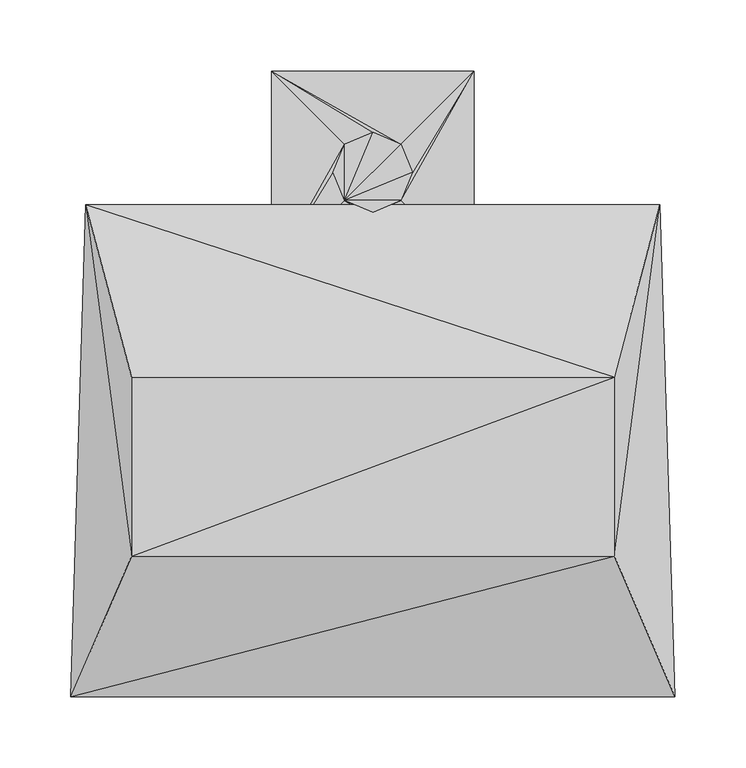
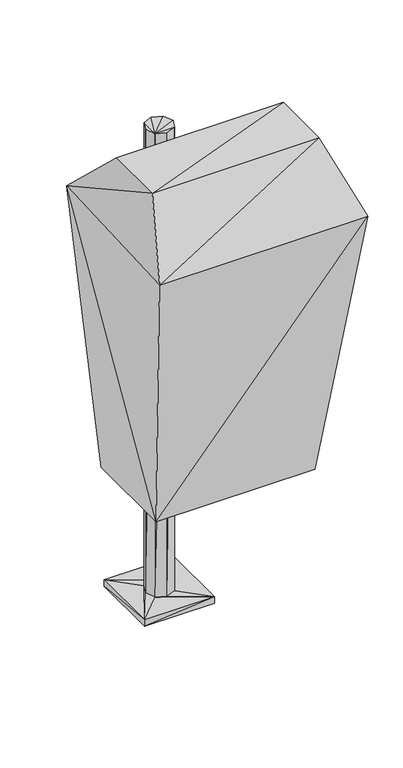
"""IFC4 building model written with IfcOpenShell, lengths in millimetres: geographic element geometry, Enscape AssetDefinition - Garbage Bin 011 : Enscape AssetDefinition - Garbage Bin 011."""

from ifc_helpers import new_model, si_unit, origin, place, context, project, spatial, faceted_brep, source, transform, mapped, element, save


def geographic_element_e7922c7f(model_context):
    return source(origin(), model_context, "Body", "Brep", [
        faceted_brep([(71.6079995, 71.6079995, 0.0), (-71.6079995, -71.6079995, 0.0), (-71.6079995, 71.6079995, 0.0), (71.6079995, -71.6079995, 0.0), (-71.6079995, -71.6079995, 13.855), (71.6079995, -71.6079995, 13.855), (-71.6079995, 71.6079995, 13.855), (71.6079995, 71.6079995, 13.855), (0.0, -28.1310007, 13.855), (19.8919997, -19.8919997, 13.855), (-19.8919997, -19.8919997, 13.855), (28.1310007, 0.0, 13.855), (19.8919997, 19.8919997, 13.855), (19.8919997, -19.8919997, 1016.2409544), (28.1310007, 0.0, 1016.2409544), (0.0, -28.1310007, 1016.2409544), (-28.1310007, 0.0, 13.855), (-19.8919997, -19.8919997, 1016.2409544), (19.8919997, 19.8919997, 1016.2409544), (0.0, 28.1310007, 1016.2409544), (-19.8919997, 19.8919997, 1016.2409544), (-28.1310007, 0.0, 1016.2409544), (-19.8919997, 19.8919997, 13.855), (0.0, 28.1310007, 13.855)], [[[0, 1, 2]], [[3, 1, 0]], [[4, 2, 1]], [[5, 1, 3]], [[4, 1, 5]], [[6, 2, 4]], [[6, 0, 2]], [[7, 3, 0]], [[7, 0, 6]], [[5, 3, 7]], [[8, 5, 9]], [[10, 5, 8]], [[5, 10, 4]], [[7, 9, 5]], [[11, 7, 12]], [[9, 7, 11]], [[6, 12, 7]], [[13, 8, 9]], [[14, 9, 11]], [[13, 9, 14]], [[15, 8, 13]], [[15, 10, 8]], [[16, 4, 10]], [[17, 16, 10]], [[17, 10, 15]], [[13, 17, 15]], [[14, 17, 13]], [[18, 17, 14]], [[14, 11, 18]], [[18, 11, 12]], [[19, 17, 18]], [[18, 12, 19]], [[20, 17, 19]], [[17, 20, 21]], [[21, 16, 17]], [[22, 4, 16]], [[21, 22, 16]], [[20, 22, 21]], [[20, 23, 22]], [[19, 23, 20]], [[19, 12, 23]], [[23, 6, 22]], [[12, 6, 23]], [[4, 22, 6]]]),
        faceted_brep([(170.502007, -144.7360069, 1092.8790569), (-202.9629946, -22.9189992, 969.7870016), (-170.502007, -144.7360069, 1092.8790569), (202.9629946, -22.9189992, 969.7870016), (170.502007, -270.931989, 1092.8790569), (213.3489996, -370.4110086, 968.7119722), (162.5470072, -76.2519985, 378.6059916), (162.5470072, -270.931989, 378.6059916), (-162.5470072, -270.931989, 378.6059916), (-213.3489996, -370.4110086, 968.7119722), (-162.5470072, -76.2519985, 378.6059916), (-170.502007, -270.931989, 1092.8790569)], [[[0, 1, 2]], [[3, 1, 0]], [[3, 4, 5]], [[0, 4, 3]], [[6, 5, 7]], [[3, 5, 6]], [[1, 8, 9]], [[10, 8, 1]], [[11, 0, 2]], [[4, 0, 11]], [[7, 10, 6]], [[8, 10, 7]], [[3, 10, 1]], [[6, 10, 3]], [[9, 4, 11]], [[5, 4, 9]], [[11, 1, 9]], [[2, 1, 11]], [[5, 8, 7]], [[9, 8, 5]]]),
    ])


if __name__ == "__main__":
    model = new_model("IFC4")
    model_context = context("Model", 3, world=origin())
    ifc_project = project(units=[si_unit("LENGTHUNIT", "METRE", prefix="MILLI")], contexts=[model_context])
    site = spatial("IfcSite", under=ifc_project)
    building = spatial("IfcBuilding", under=site)
    placement = place(None, origin())
    geographic_element_shape = geographic_element_e7922c7f(model_context)
    element("IfcGeographicElement", 1, ObjectType="Enscape AssetDefinition - Garbage Bin 011 : Enscape AssetDefinition - Garbage Bin 011", at=placement, inside=building, context=model_context, shape_type="MappedRepresentation", body=[
        mapped(geographic_element_shape, transform((0.0, 0.0, 0.0), x_axis=(1.0, 0.0, 0.0), y_axis=(0.0, 1.0, 0.0), z_axis=(0.0, 0.0, 1.0))),
    ])
    save(model, "model.ifc")

# Revit data of these elements
# Type "Enscape AssetDefinition - Garbage Bin 011 : Enscape AssetDefinition - Garbage Bin 011"
#   EnscapeAssetSource = "REMOTE"
#   EnscapeAssetId = "efc4cba8-a6d2-4f52-9618-2b508df8dd30"
#   Height = 1.092879 m
#   EnscapeNativeAssetHeight = 1.092879 m
#   Default Elevation = 0
